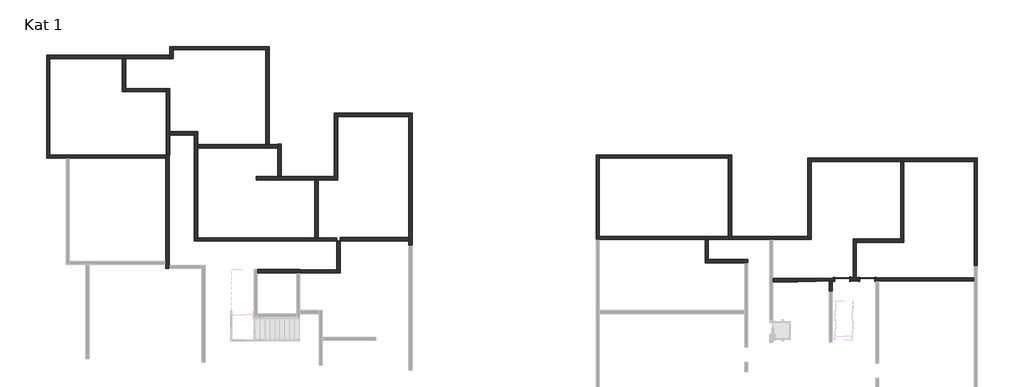
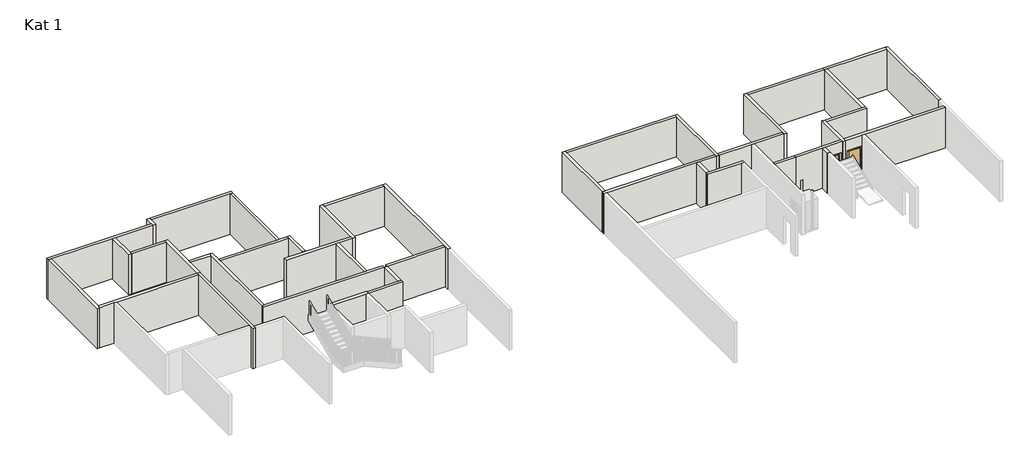
# One storey, part 2 of 3: 43 walls, 2 doors.
"""IFC4 building model written with IfcOpenShell, lengths in millimetres."""

import ifcopenshell
import ifcopenshell.guid

model = None  # the IFC model being written
_history = None  # IfcOwnerHistory: only IFC2X3 demands one
_inside = {}  # id of a spatial element -> (the spatial element, [elements in it])
_under = {}  # id of a project, library or spatial element -> (it, [spatial elements below it])
_declared = {}  # id of a project -> (the project, [libraries it declares])
_typed = {}  # id of a type object -> (the type object, [elements of that type])
_made_of = {}  # id of a material, layer set ... -> (it, [elements and type objects made of it])


def new_model(schema):
    """Start an empty IFC model of exactly this schema.

    Asked for "IFC4X3", IfcOpenShell would pick the latest addendum, in which some entities
    have other attributes; the version numbers below select the first issue.
    IFC2X3 requires an IfcOwnerHistory on every rooted entity: one is made here for all.
    """
    global model, _history
    if schema == "IFC4X3":
        model = ifcopenshell.file(schema_version=(4, 3, 0, 0))
    else:
        model = ifcopenshell.file(schema=schema)
    _inside.clear()
    _under.clear()
    _declared.clear()
    _typed.clear()
    _made_of.clear()
    _history = None
    if model.schema == "IFC2X3":
        org = make("IfcOrganization", Name="unknown")
        user = make(
            "IfcPersonAndOrganization",
            ThePerson=make("IfcPerson", FamilyName="unknown"),
            TheOrganization=org,
        )
        app = make(
            "IfcApplication",
            ApplicationDeveloper=org,
            Version="unknown",
            ApplicationFullName="unknown",
            ApplicationIdentifier="unknown",
        )
        _history = make(
            "IfcOwnerHistory",
            OwningUser=user,
            OwningApplication=app,
            ChangeAction="ADDED",
            CreationDate=0,
        )
    return model


def make(cls, **values):
    """One entity of the class cls with the attributes given. An attribute that is None is left unset."""
    return model.create_entity(
        cls, **{name: value for name, value in values.items() if value is not None}
    )


def rooted(cls, **values):
    """An entity with a GlobalId (a new one), such as an element, a storey or a relation."""
    return make(cls, GlobalId=ifcopenshell.guid.new(), OwnerHistory=_history, **values)


def si_unit(unit_type, name, prefix=None):
    """IfcSIUnit, for example si_unit("LENGTHUNIT", "METRE", prefix="MILLI")."""
    return make("IfcSIUnit", UnitType=unit_type, Prefix=prefix, Name=name)


def assignment(units):
    """IfcUnitAssignment: the units of a project."""
    return None if units is None else make("IfcUnitAssignment", Units=units)


def point(xyz):
    """IfcCartesianPoint."""
    return None if xyz is None else make("IfcCartesianPoint", Coordinates=xyz)


def direction(xyz):
    """IfcDirection."""
    return None if xyz is None else make("IfcDirection", DirectionRatios=xyz)


def frame(location, z_axis=None, x_axis=None):
    """IfcAxis2Placement3D, a coordinate frame: its origin and axes. An axis left out is left unset."""
    return make(
        "IfcAxis2Placement3D",
        Location=point(location),
        Axis=direction(z_axis),
        RefDirection=direction(x_axis),
    )


def origin():
    """The frame at (0, 0, 0) with its axes left unset."""
    return frame((0.0, 0.0, 0.0))


def origin_with_axes():
    """The frame at (0, 0, 0) with the z axis (0, 0, 1) and the x axis (1, 0, 0) written out."""
    return frame((0.0, 0.0, 0.0), z_axis=(0.0, 0.0, 1.0), x_axis=(1.0, 0.0, 0.0))


def place(relative_to, where):
    """IfcLocalPlacement: puts the frame where relative to a parent placement (None: the world)."""
    return make(
        "IfcLocalPlacement", PlacementRelTo=relative_to, RelativePlacement=where
    )


def context(
    kind, dimensions, precision=None, world=None, true_north=None, identifier=None
):
    """IfcGeometricRepresentationContext, for example the 3D "Model" context."""
    return make(
        "IfcGeometricRepresentationContext",
        ContextIdentifier=identifier,
        ContextType=kind,
        CoordinateSpaceDimension=dimensions,
        Precision=precision,
        WorldCoordinateSystem=world,
        TrueNorth=true_north,
    )


def project(units=None, contexts=None):
    """IfcProject with its units and contexts."""
    return rooted(
        "IfcProject",
        Name="project",
        RepresentationContexts=contexts,
        UnitsInContext=assignment(units),
    )


def spatial(cls, under=None, at=None, **own):
    """A site, building, storey or space (cls), placed at a placement, below another one or the project."""
    s = rooted(cls, ObjectPlacement=at, **own)
    if under is not None:
        _under.setdefault(under.id(), (under, []))[1].append(s)
    return s


def polyline(points):
    """IfcPolyline through the points."""
    return make("IfcPolyline", Points=[point(p) for p in points])


def outline(outer, holes=None, kind="AREA"):
    """IfcArbitraryClosedProfileDef: a profile drawn as a closed curve; with holes, ...WithVoids."""
    if holes is None:
        return make("IfcArbitraryClosedProfileDef", ProfileType=kind, OuterCurve=outer)
    return make(
        "IfcArbitraryProfileDefWithVoids",
        ProfileType=kind,
        OuterCurve=outer,
        InnerCurves=holes,
    )


def extrude(swept, where, along, depth):
    """IfcExtrudedAreaSolid: the profile swept, set in the frame where, extruded along a direction by depth."""
    return make(
        "IfcExtrudedAreaSolid",
        SweptArea=swept,
        Position=where,
        ExtrudedDirection=direction(along),
        Depth=depth,
    )


def faces_of(points, faces, orient=None, outer=None):
    """IfcFace entities. A face is a list of loops; a loop is a list of indices into points, from 0.

    orient and outer hold one flag for each loop. By default every Orientation is true, the
    first loop of a face is its IfcFaceOuterBound and the others are IfcFaceBound.
    """
    made = []
    for i, loops in enumerate(faces):
        bounds = []
        for j, loop in enumerate(loops):
            is_outer = j == 0 if outer is None else outer[i][j]
            bounds.append(
                make(
                    "IfcFaceOuterBound" if is_outer else "IfcFaceBound",
                    Bound=make("IfcPolyLoop", Polygon=[points[k] for k in loop]),
                    Orientation=True if orient is None else orient[i][j],
                )
            )
        made.append(make("IfcFace", Bounds=bounds))
    return made


def faceted_brep(points, faces, orient=None, outer=None, voids=None):
    """IfcFacetedBrep: a solid bounded by flat faces; with voids (closed shells), ...WithVoids."""
    shared = [point(p) for p in points]
    hull = make("IfcClosedShell", CfsFaces=faces_of(shared, faces, orient, outer))
    if voids is None:
        return make("IfcFacetedBrep", Outer=hull)
    return make(
        "IfcFacetedBrepWithVoids",
        Outer=hull,
        Voids=[
            make(cls, CfsFaces=faces_of(shared, fs, o, b)) for cls, fs, o, b in voids
        ],
    )


def shape(context_of_items, identifier, shape_type, items):
    """IfcShapeRepresentation: the items that make up one representation, for example the "Body"."""
    return make(
        "IfcShapeRepresentation",
        ContextOfItems=context_of_items,
        RepresentationIdentifier=identifier,
        RepresentationType=shape_type,
        Items=items,
    )


def source(mapping_origin, context_of_items, identifier, shape_type, items):
    """IfcRepresentationMap: a shape defined once, which mapped items show again and again."""
    return make(
        "IfcRepresentationMap",
        MappingOrigin=mapping_origin,
        MappedRepresentation=shape(context_of_items, identifier, shape_type, items),
    )


def transform(
    local_origin,
    x_axis=None,
    y_axis=None,
    z_axis=None,
    scale=None,
    scale2=None,
    scale3=None,
    uniform=True,
):
    """IfcCartesianTransformationOperator3D, or its non-uniform kind. x_axis, y_axis, z_axis: its Axis1, 2, 3."""
    if uniform:
        return make(
            "IfcCartesianTransformationOperator3D",
            Axis1=direction(x_axis),
            Axis2=direction(y_axis),
            LocalOrigin=point(local_origin),
            Scale=scale,
            Axis3=direction(z_axis),
        )
    return make(
        "IfcCartesianTransformationOperator3DnonUniform",
        Axis1=direction(x_axis),
        Axis2=direction(y_axis),
        LocalOrigin=point(local_origin),
        Scale=scale,
        Axis3=direction(z_axis),
        Scale2=scale2,
        Scale3=scale3,
    )


def mapped(mapping_source, mapping_target):
    """IfcMappedItem: shows the shape of a source again, moved by a transform."""
    return make(
        "IfcMappedItem", MappingSource=mapping_source, MappingTarget=mapping_target
    )


def made_of(thing, what):
    """Note that an element or type object is made of a material, layer set ...; save() writes the relation."""
    if what is not None:
        _made_of.setdefault(what.id(), (what, []))[1].append(thing)
    return thing


def element(
    cls,
    number,
    at=None,
    inside=None,
    cuts=None,
    type_object=None,
    material=None,
    context=None,
    identifier="Body",
    shape_type=None,
    held_by="IfcProductDefinitionShape",
    body=None,
    shapes=None,
    **own,
):
    """One element of the class cls, such as IfcWall. Its Tag is "e" and its number.

    at: its placement. inside: the storey or other place that contains it. cuts: it is an
    opening in that element (IfcRelVoidsElement). A single representation is given by context,
    identifier, shape_type and body (its items); several are given by shapes. held_by: the class
    of the entity that holds the representations. save() writes the other relations.
    """
    e = rooted(cls, Tag="e%d" % number, ObjectPlacement=at, **own)
    if body is not None:
        shapes = [shape(context, identifier, shape_type, body)]
    if shapes is not None:
        e.Representation = make(held_by, Representations=shapes)
    if inside is not None:
        _inside.setdefault(inside.id(), (inside, []))[1].append(e)
    if cuts is not None:
        rooted(
            "IfcRelVoidsElement", RelatingBuildingElement=cuts, RelatedOpeningElement=e
        )
    if type_object is not None:
        _typed.setdefault(type_object.id(), (type_object, []))[1].append(e)
    return made_of(e, material)


def aggregate(whole, parts):
    """IfcRelAggregates: a whole, such as a stair, and the parts it consists of."""
    return rooted("IfcRelAggregates", RelatingObject=whole, RelatedObjects=parts)


def save(model, path):
    """Write the relations noted so far, then the file.

    IfcRelAggregates (storeys below a building ...), IfcRelContainedInSpatialStructure (elements
    in a storey), IfcRelDefinesByType, IfcRelAssociatesMaterial and IfcRelDeclares: one each for
    every whole, place, type object, material and project.
    """
    for whole, parts in _under.values():
        aggregate(whole, parts)
    for where, things in _inside.values():
        rooted(
            "IfcRelContainedInSpatialStructure",
            RelatedElements=things,
            RelatingStructure=where,
        )
    for kind, things in _typed.values():
        rooted("IfcRelDefinesByType", RelatedObjects=things, RelatingType=kind)
    for what, things in _made_of.values():
        rooted("IfcRelAssociatesMaterial", RelatedObjects=things, RelatingMaterial=what)
    for by, libraries in _declared.values():
        rooted("IfcRelDeclares", RelatingContext=by, RelatedDefinitions=libraries)
    model.write(path)


def m_single_flush_0915_x_2134mm_727434cd(model_context):
    return source(origin(), model_context, "Body", "SweptSolid", [
        extrude(outline(polyline([(2210.0, -533.5), (0.0, -533.5), (0.0, -457.5), (2134.0, -457.5), (2134.0, 457.5), (0.0, 457.5), (0.0, 533.5), (2210.0, 533.5), (2210.0, -533.5)])), frame((0.0, -125.0, 0.0), z_axis=(0.0, 1.0, 0.0), x_axis=(0.0, 0.0, 1.0)), (0.0, 0.0, 1.0), 25.0),
        extrude(outline(polyline([(2210.0, 533.5), (2210.0, -533.5), (0.0, -533.5), (0.0, -457.5), (2134.0, -457.5), (2134.0, 457.5), (0.0, 457.5), (0.0, 533.5), (2210.0, 533.5)])), frame((0.0, 100.0, 0.0), z_axis=(0.0, 1.0, 0.0), x_axis=(0.0, 0.0, 1.0)), (0.0, 0.0, 1.0), 25.0),
        extrude(outline(polyline([(457.5, -49.0), (457.5, -100.0), (-457.5, -100.0), (-457.5, -49.0), (457.5, -49.0)])), origin_with_axes(), (0.0, 0.0, 1.0), 2134.0),
    ])


def m_single_flush_0915_x_2134mm_6a9e8738(model_context):
    return source(origin(), model_context, "Body", "SweptSolid", [
        extrude(outline(polyline([(2210.0, -533.5), (0.0, -533.5), (0.0, -457.5), (2134.0, -457.5), (2134.0, 457.5), (0.0, 457.5), (0.0, 533.5), (2210.0, 533.5), (2210.0, -533.5)])), frame((0.0, 100.0, 0.0), z_axis=(0.0, 1.0, 0.0), x_axis=(0.0, 0.0, 1.0)), (0.0, 0.0, 1.0), 25.0),
        extrude(outline(polyline([(2210.0, 533.5), (2210.0, -533.5), (0.0, -533.5), (0.0, -457.5), (2134.0, -457.5), (2134.0, 457.5), (0.0, 457.5), (0.0, 533.5), (2210.0, 533.5)])), frame((0.0, -125.0, 0.0), z_axis=(0.0, 1.0, 0.0), x_axis=(0.0, 0.0, 1.0)), (0.0, 0.0, 1.0), 25.0),
        extrude(outline(polyline([(457.5, 49.0), (-457.5, 49.0), (-457.5, 100.0), (457.5, 100.0), (457.5, 49.0)])), origin_with_axes(), (0.0, 0.0, 1.0), 2134.0),
    ])


model = new_model("IFC4")

# Units and contexts
model_context = context("Model", 3, world=origin())
ifc_project = project(units=[si_unit("LENGTHUNIT", "METRE", prefix="MILLI")], contexts=[model_context])

# Site, building, storey
site = spatial("IfcSite", under=ifc_project)
building = spatial("IfcBuilding", under=site)
storey = spatial("IfcBuildingStorey", under=building, Name="Kat 1", Elevation=3000.0)

# Doors
placement = place(None, origin())
m_single_flush_0915_x_2134mm_shape = m_single_flush_0915_x_2134mm_727434cd(model_context)
element("IfcDoor", 1, ObjectType="M_Single-Flush : 0915 x 2134mm", at=placement, inside=storey, context=model_context, shape_type="MappedRepresentation", body=[
    mapped(m_single_flush_0915_x_2134mm_shape, transform((23647.336337, 521.2707349, 3000.0), x_axis=(-1.0, 0.0, 0.0), y_axis=(0.0, -1.0, 0.0), z_axis=(0.0, 0.0, 1.0))),
])
m_single_flush_0915_x_2134mm_2_shape = m_single_flush_0915_x_2134mm_6a9e8738(model_context)
element("IfcDoor", 2, ObjectType="M_Single-Flush : 0915 x 2134mm", at=placement, inside=storey, context=model_context, shape_type="MappedRepresentation", body=[
    mapped(m_single_flush_0915_x_2134mm_2_shape, transform((22134.1969486, 528.0657675, 3000.0), x_axis=(0.9998476951563913, 0.01745240643728349, 0.0), y_axis=(-0.01745240643728349, 0.9998476951563913, 0.0), z_axis=(0.0, 0.0, 1.0))),
])

# Walls
element("IfcWall", 3, ObjectType="Generic - 200mm", at=placement, inside=storey, context=model_context, shape_type="Brep", body=[
    faceted_brep([(25649.836337, 7621.2707349, 3000.0), (25849.836337, 7621.2707349, 3000.0), (30068.3425199, 7621.2707349, 3000.0), (30068.3425199, 7621.2707349, 6000.0), (25849.836337, 7621.2707349, 6000.0), (25649.836337, 7621.2707349, 6000.0), (25649.836337, 7821.2707349, 3000.0), (25649.836337, 7821.2707349, 6000.0), (30068.3425199, 7821.2707349, 6000.0), (30068.3425199, 7821.2707349, 3000.0), (30068.3425199, 7819.475628, 3000.0)], [[[0, 1, 2, 3, 4, 5]], [[6, 7, 8, 9]], [[2, 1, 0, 6, 9, 10]], [[5, 4, 3, 8, 7]], [[0, 5, 7, 6]], [[3, 2, 10, 9, 8]]]),
])
element("IfcWall", 4, ObjectType="Generic - 200mm", at=placement, inside=storey, context=model_context, shape_type="Brep", body=[
    faceted_brep([(30068.3425199, 7821.2707349, 3000.0), (30068.3425199, 7819.475628, 3000.0), (30068.3425199, 7621.2707349, 3000.0), (30068.3425199, 1319.475628, 3000.0), (30068.3425199, 1319.475628, 6000.0), (30068.3425199, 7621.2707349, 6000.0), (30068.3425199, 7821.2707349, 6000.0), (30268.3425199, 7821.2707349, 3000.0), (30268.3425199, 7821.2707349, 6000.0), (30268.3425199, 1319.475628, 6000.0), (30268.3425199, 1319.475628, 3000.0), (30268.3425199, 7819.475628, 3000.0), (30068.8612349, 1319.475628, 3000.0), (30068.8612349, 1319.475628, 6000.0)], [[[0, 1, 2, 3, 4, 5, 6]], [[7, 8, 9, 10, 11]], [[3, 2, 1, 0, 7, 11, 10, 12]], [[4, 3, 12, 10, 9, 13]], [[6, 5, 4, 13, 9, 8]], [[0, 6, 8, 7]]]),
])
element("IfcWall", 5, ObjectType="Generic - 200mm", at=placement, inside=storey, context=model_context, shape_type="Brep", body=[
    faceted_brep([(21549.836337, -200.524372, 3000.0), (21549.836337, 379.475628, 3000.0), (21549.836337, 417.8504823, 3000.0), (21549.836337, 417.8504823, 6000.0), (21549.836337, -200.524372, 6000.0), (21349.836337, -200.524372, 3000.0), (21349.836337, -200.524372, 6000.0), (21349.836337, 414.3594693, 6000.0), (21349.836337, 414.3594693, 3000.0), (21349.836337, 379.475628, 3000.0)], [[[0, 1, 2, 3, 4]], [[5, 6, 7, 8, 9]], [[2, 1, 0, 5, 9, 8]], [[4, 3, 7, 6]], [[0, 4, 6, 5]], [[3, 2, 8, 7]]]),
])
element("IfcWall", 6, ObjectType="Generic - 200mm", at=placement, inside=storey, context=model_context, shape_type="Brep", body=[
    faceted_brep([(20268.8612349, 7621.2707349, 3000.0), (25649.836337, 7621.2707349, 3000.0), (25649.836337, 7621.2707349, 6000.0), (20268.8612349, 7621.2707349, 6000.0), (20268.8612349, 7821.2707349, 3000.0), (20268.8612349, 7821.2707349, 6000.0), (25649.836337, 7821.2707349, 6000.0), (25649.836337, 7821.2707349, 3000.0), (20268.8612349, 7819.475628, 3000.0)], [[[0, 1, 2, 3]], [[4, 5, 6, 7]], [[1, 0, 8, 4, 7]], [[3, 2, 6, 5]], [[2, 1, 7, 6]], [[0, 3, 5, 4, 8]]]),
])
element("IfcWall", 7, ObjectType="Generic - 200mm", at=placement, inside=storey, context=model_context, shape_type="Brep", body=[
    faceted_brep([(22989.836337, 421.2707349, 3000.0), (22989.836337, 621.2707349, 3000.0), (22989.836337, 2756.2707349, 3000.0), (22989.836337, 2956.2707349, 3000.0), (22989.836337, 2956.2707349, 6000.0), (22989.836337, 2756.2707349, 6000.0), (22989.836337, 621.2707349, 6000.0), (22989.836337, 421.2707349, 6000.0), (22789.836337, 421.2707349, 3000.0), (22789.836337, 421.2707349, 6000.0), (22789.836337, 439.4947628, 6000.0), (22789.836337, 639.5252284, 6000.0), (22789.836337, 2956.2707349, 6000.0), (22789.836337, 2956.2707349, 3000.0), (22789.836337, 639.5252284, 3000.0), (22789.836337, 439.4947628, 3000.0)], [[[0, 1, 2, 3, 4, 5, 6, 7]], [[8, 9, 10, 11, 12, 13, 14, 15]], [[3, 2, 1, 0, 8, 15, 14, 13]], [[7, 6, 5, 4, 12, 11, 10, 9]], [[4, 3, 13, 12]], [[0, 7, 9, 8]]]),
])
element("IfcWall", 8, ObjectType="Generic - 200mm", at=placement, inside=storey, context=model_context, shape_type="Brep", body=[
    faceted_brep([(13888.8612349, 1521.4230978, 3000.0), (16270.6041014, 1521.4230978, 3000.0), (16470.6041014, 1521.4230978, 3000.0), (16470.6041014, 1521.4230978, 6000.0), (16270.6041014, 1521.4230978, 6000.0), (13888.8612349, 1521.4230978, 6000.0), (13888.8612349, 1721.4230978, 3000.0), (13888.8612349, 1721.4230978, 6000.0), (14088.8612349, 1721.4230978, 6000.0), (16470.6041014, 1721.4230978, 6000.0), (16470.6041014, 1721.4230978, 3000.0), (14088.8612349, 1721.4230978, 3000.0)], [[[0, 1, 2, 3, 4, 5]], [[6, 7, 8, 9, 10, 11]], [[2, 1, 0, 6, 11, 10]], [[5, 4, 3, 9, 8, 7]], [[0, 5, 7, 6]], [[3, 2, 10, 9]]]),
])
element("IfcWall", 9, ObjectType="Generic - 200mm", at=placement, inside=storey, context=model_context, shape_type="Brep", body=[
    faceted_brep([(20068.8612349, 7821.2707349, 3000.0), (20068.8612349, 7819.475628, 3000.0), (20068.8612349, 3121.2707349, 3000.0), (20068.8612349, 2921.2707349, 3000.0), (20068.8612349, 2921.2707349, 6000.0), (20068.8612349, 3121.2707349, 6000.0), (20068.8612349, 7821.2707349, 6000.0), (20268.8612349, 7821.2707349, 3000.0), (20268.8612349, 7821.2707349, 6000.0), (20268.8612349, 7621.2707349, 6000.0), (20268.8612349, 2921.2707349, 6000.0), (20268.8612349, 2921.2707349, 3000.0), (20268.8612349, 7621.2707349, 3000.0), (20268.8612349, 7819.475628, 3000.0)], [[[0, 1, 2, 3, 4, 5, 6]], [[7, 8, 9, 10, 11, 12, 13]], [[3, 2, 1, 0, 7, 13, 12, 11]], [[6, 5, 4, 10, 9, 8]], [[0, 6, 8, 7]], [[4, 3, 11, 10]]]),
])
element("IfcWall", 10, ObjectType="Generic - 200mm", at=placement, inside=storey, context=model_context, shape_type="Brep", body=[
    faceted_brep([(30068.8612349, 421.2707349, 6000.0), (24348.8612349, 421.2707349, 6000.0), (24148.8612349, 421.2707349, 6000.0), (22989.836337, 421.2707349, 6000.0), (22989.836337, 421.2707349, 3000.0), (23189.836337, 421.2707349, 3000.0), (23189.836337, 421.2707349, 5134.0), (24104.836337, 421.2707349, 5134.0), (24104.836337, 421.2707349, 3000.0), (24148.8612349, 421.2707349, 3000.0), (24348.8612349, 421.2707349, 3000.0), (30068.8612349, 421.2707349, 3000.0), (22989.836337, 621.2707349, 6000.0), (30068.8612349, 621.2707349, 6000.0), (30068.8612349, 621.2707349, 3000.0), (24104.836337, 621.2707349, 3000.0), (24104.836337, 621.2707349, 5134.0), (23189.836337, 621.2707349, 5134.0), (23189.836337, 621.2707349, 3000.0), (22989.836337, 621.2707349, 3000.0)], [[[0, 1, 2, 3, 4, 5, 6, 7, 8, 9, 10, 11]], [[12, 13, 14, 15, 16, 17, 18, 19]], [[14, 11, 10, 9, 8, 15]], [[4, 19, 18, 5]], [[3, 2, 1, 0, 13, 12]], [[0, 11, 14, 13]], [[17, 6, 5, 18]], [[7, 16, 15, 8]], [[16, 7, 6, 17]], [[19, 4, 3, 12]]]),
])
element("IfcWall", 11, ObjectType="Generic - 200mm", at=placement, inside=storey, context=model_context, shape_type="SweptSolid", body=[
    extrude(outline(polyline([(17970.6041014, 581.2707349), (19452.4386392, 581.2707349), (19454.1840127, 381.2707349), (17970.6041014, 381.2707349), (17970.6041014, 581.2707349)])), frame((0.0, 0.0, 3000.0), z_axis=(0.0, 0.0, 1.0), x_axis=(1.0, 0.0, 0.0)), (0.0, 0.0, 1.0), 3000.0),
])
element("IfcWall", 12, ObjectType="Generic - 200mm", at=placement, inside=storey, context=model_context, shape_type="Brep", body=[
    faceted_brep([(19452.4386392, 581.2707349, 6000.0), (22789.836337, 639.5252284, 6000.0), (22789.836337, 639.5252284, 3000.0), (22589.8820285, 636.035013, 3000.0), (22589.8820285, 636.035013, 5134.0), (21675.0213874, 620.0660611, 5134.0), (21675.0213874, 620.0660611, 3000.0), (19452.4386392, 581.2707349, 3000.0), (22789.836337, 439.4947628, 6000.0), (21549.836337, 417.8504823, 6000.0), (21349.836337, 414.3594693, 6000.0), (19454.1840127, 381.2707349, 6000.0), (19454.1840127, 381.2707349, 3000.0), (21349.836337, 414.3594693, 3000.0), (21549.836337, 417.8504823, 3000.0), (21678.5118687, 420.0965221, 3000.0), (21678.5118687, 420.0965221, 5134.0), (22593.3725098, 436.0654739, 5134.0), (22593.3725098, 436.0654739, 3000.0), (22789.836337, 439.4947628, 3000.0)], [[[0, 1, 2, 3, 4, 5, 6, 7]], [[8, 9, 10, 11, 12, 13, 14, 15, 16, 17, 18, 19]], [[2, 19, 18, 3]], [[12, 7, 6, 15, 14, 13]], [[1, 0, 11, 10, 9, 8]], [[17, 4, 3, 18]], [[5, 16, 15, 6]], [[16, 5, 4, 17]], [[2, 1, 8, 19]], [[11, 0, 7, 12]]]),
])
element("IfcWall", 13, ObjectType="Generic - 200mm", at=placement, inside=storey, context=model_context, shape_type="Brep", body=[
    faceted_brep([(22989.836337, 2756.2707349, 3000.0), (25849.836337, 2756.2707349, 3000.0), (25849.836337, 2756.2707349, 6000.0), (22989.836337, 2756.2707349, 6000.0), (22989.836337, 2956.2707349, 3000.0), (22989.836337, 2956.2707349, 6000.0), (25649.836337, 2956.2707349, 6000.0), (25849.836337, 2956.2707349, 6000.0), (25849.836337, 2956.2707349, 3000.0), (25649.836337, 2956.2707349, 3000.0)], [[[0, 1, 2, 3]], [[4, 5, 6, 7, 8, 9]], [[1, 0, 4, 9, 8]], [[3, 2, 7, 6, 5]], [[2, 1, 8, 7]], [[0, 3, 5, 4]]]),
])
element("IfcWall", 14, ObjectType="Generic - 200mm", at=placement, inside=storey, context=model_context, shape_type="SweptSolid", body=[
    extrude(outline(polyline([(25849.836337, 7621.2707349), (25849.836337, 2956.2707349), (25649.836337, 2956.2707349), (25649.836337, 7621.2707349), (25849.836337, 7621.2707349)])), frame((0.0, 0.0, 3000.0), z_axis=(0.0, 0.0, 1.0), x_axis=(1.0, 0.0, 0.0)), (0.0, 0.0, 1.0), 3000.0),
])
element("IfcWall", 15, ObjectType="Generic - 200mm", at=placement, inside=storey, context=model_context, shape_type="Brep", body=[
    faceted_brep([(-10469.8304233, 1122.632394, 3000.0), (-13026.101437, 1122.632394, 3000.0), (-13026.101437, 1122.632394, 6000.0), (-10469.8304233, 1122.632394, 6000.0), (-10469.8304233, 922.632394, 3000.0), (-10469.8304233, 922.632394, 6000.0), (-10669.8304233, 922.632394, 6000.0), (-13026.101437, 922.632394, 6000.0), (-13026.101437, 922.632394, 3000.0), (-10669.8304233, 922.632394, 3000.0), (-10469.8304233, 1102.632394, 3000.0), (-13026.101437, 1120.8372871, 3000.0), (-10469.8304233, 1102.632394, 6000.0)], [[[0, 1, 2, 3]], [[4, 5, 6, 7, 8, 9]], [[1, 0, 10, 4, 9, 8, 11]], [[3, 2, 7, 6, 5, 12]], [[0, 3, 12, 5, 4, 10]], [[2, 1, 11, 8, 7]]]),
])
element("IfcWall", 16, ObjectType="Generic - 200mm", at=placement, inside=storey, context=model_context, shape_type="Brep", body=[
    faceted_brep([(-18289.8304233, 8014.6351355, 3000.0), (-18289.8304233, 9214.6351355, 3000.0), (-18289.8304233, 9414.6351355, 3000.0), (-18289.8304233, 12014.6351355, 3000.0), (-18289.8304233, 12014.6351355, 6000.0), (-18289.8304233, 9414.6351355, 6000.0), (-18289.8304233, 9214.6351355, 6000.0), (-18289.8304233, 8014.6351355, 6000.0), (-18489.8304233, 8014.6351355, 3000.0), (-18489.8304233, 8014.6351355, 6000.0), (-18489.8304233, 11814.6351355, 6000.0), (-18489.8304233, 12014.6351355, 6000.0), (-18489.8304233, 12014.6351355, 3000.0), (-18489.8304233, 11814.6351355, 3000.0), (-18323.9741722, 8014.6351355, 3000.0), (-18323.9741722, 8014.6351355, 6000.0)], [[[0, 1, 2, 3, 4, 5, 6, 7]], [[8, 9, 10, 11, 12, 13]], [[3, 2, 1, 0, 14, 8, 13, 12]], [[7, 6, 5, 4, 11, 10, 9, 15]], [[0, 7, 15, 9, 8, 14]], [[4, 3, 12, 11]]]),
])
element("IfcWall", 17, ObjectType="Generic - 200mm", at=placement, inside=storey, context=model_context, shape_type="Brep", body=[
    faceted_brep([(15288.8612349, 3120.535295, 3000.0), (7543.716007, 3120.535295, 3000.0), (7343.716007, 3120.535295, 3000.0), (7343.716007, 3120.535295, 6000.0), (7543.716007, 3120.535295, 6000.0), (15288.8612349, 3120.535295, 6000.0), (15288.8612349, 2920.535295, 3000.0), (15288.8612349, 2920.535295, 6000.0), (14088.8612349, 2920.535295, 6000.0), (13888.8612349, 2920.535295, 6000.0), (7543.716007, 2920.535295, 6000.0), (7343.716007, 2920.535295, 6000.0), (7343.716007, 2920.535295, 3000.0), (7543.716007, 2920.535295, 3000.0), (13888.8612349, 2920.535295, 3000.0), (14088.8612349, 2920.535295, 3000.0), (7343.716007, 3020.535295, 3000.0)], [[[0, 1, 2, 3, 4, 5]], [[6, 7, 8, 9, 10, 11, 12, 13, 14, 15]], [[2, 1, 0, 6, 15, 14, 13, 12, 16]], [[5, 4, 3, 11, 10, 9, 8, 7]], [[3, 2, 16, 12, 11]], [[0, 5, 7, 6]]]),
])
element("IfcWall", 18, ObjectType="Generic - 200mm", at=placement, inside=storey, context=model_context, shape_type="Brep", body=[
    faceted_brep([(-12326.101437, 14542.632394, 3000.0), (-18089.8304233, 14542.632394, 3000.0), (-18089.8304233, 14542.632394, 6000.0), (-12326.101437, 14542.632394, 6000.0), (-12326.101437, 14342.632394, 3000.0), (-12326.101437, 14342.632394, 6000.0), (-12526.101437, 14342.632394, 6000.0), (-18089.8304233, 14342.632394, 6000.0), (-18089.8304233, 14342.632394, 3000.0), (-12526.101437, 14342.632394, 3000.0), (-12326.101437, 14540.8372871, 3000.0), (-18089.8304233, 14540.8372871, 3000.0)], [[[0, 1, 2, 3]], [[4, 5, 6, 7, 8, 9]], [[1, 0, 10, 4, 9, 8, 11]], [[3, 2, 7, 6, 5]], [[2, 1, 11, 8, 7]], [[0, 3, 5, 4, 10]]]),
])
element("IfcWall", 19, ObjectType="Generic - 200mm", at=placement, inside=storey, context=model_context, shape_type="Brep", body=[
    faceted_brep([(-25701.4369496, 13814.6351355, 3000.0), (-25701.4369496, 13812.8400285, 3000.0), (-25701.4369496, 7814.6351355, 3000.0), (-25701.4369496, 7814.6351355, 6000.0), (-25701.4369496, 13814.6351355, 6000.0), (-25501.4369496, 13814.6351355, 3000.0), (-25501.4369496, 13814.6351355, 6000.0), (-25501.4369496, 8014.6351355, 6000.0), (-25501.4369496, 7814.6351355, 6000.0), (-25501.4369496, 7814.6351355, 3000.0), (-25501.4369496, 8014.6351355, 3000.0), (-25501.4369496, 13812.8400285, 3000.0)], [[[0, 1, 2, 3, 4]], [[5, 6, 7, 8, 9, 10, 11]], [[2, 1, 0, 5, 11, 10, 9]], [[4, 3, 8, 7, 6]], [[3, 2, 9, 8]], [[0, 4, 6, 5]]]),
])
element("IfcWall", 20, ObjectType="Generic - 200mm", at=placement, inside=storey, context=model_context, shape_type="Brep", body=[
    faceted_brep([(-25501.4369496, 7814.6351355, 3000.0), (-24523.9741722, 7814.6351355, 3000.0), (-24323.9741722, 7814.6351355, 3000.0), (-18523.9741722, 7814.6351355, 3000.0), (-18523.9741722, 7814.6351355, 6000.0), (-24323.9741722, 7814.6351355, 6000.0), (-24523.9741722, 7814.6351355, 6000.0), (-25501.4369496, 7814.6351355, 6000.0), (-25501.4369496, 8014.6351355, 3000.0), (-25501.4369496, 8014.6351355, 6000.0), (-18523.9741722, 8014.6351355, 6000.0), (-18523.9741722, 8014.6351355, 3000.0), (-25501.4369496, 8012.8400285, 3000.0)], [[[0, 1, 2, 3, 4, 5, 6, 7]], [[8, 9, 10, 11]], [[3, 2, 1, 0, 12, 8, 11]], [[7, 6, 5, 4, 10, 9]], [[4, 3, 11, 10]], [[0, 7, 9, 8, 12]]]),
])
element("IfcWall", 21, ObjectType="Generic - 200mm", at=placement, inside=storey, context=model_context, shape_type="Brep", body=[
    faceted_brep([(-18289.8304233, 14014.6351355, 3000.0), (-25701.4369496, 14014.6351355, 3000.0), (-25701.4369496, 14014.6351355, 6000.0), (-18289.8304233, 14014.6351355, 6000.0), (-18289.8304233, 13814.6351355, 3000.0), (-18289.8304233, 13814.6351355, 6000.0), (-20949.8304233, 13814.6351355, 6000.0), (-21149.8304233, 13814.6351355, 6000.0), (-25501.4369496, 13814.6351355, 6000.0), (-25701.4369496, 13814.6351355, 6000.0), (-25701.4369496, 13814.6351355, 3000.0), (-25501.4369496, 13814.6351355, 3000.0), (-21149.8304233, 13814.6351355, 3000.0), (-20949.8304233, 13814.6351355, 3000.0), (-18289.8304233, 14012.8400285, 3000.0), (-25701.4369496, 14012.8400285, 3000.0)], [[[0, 1, 2, 3]], [[4, 5, 6, 7, 8, 9, 10, 11, 12, 13]], [[1, 0, 14, 4, 13, 12, 11, 10, 15]], [[3, 2, 9, 8, 7, 6, 5]], [[2, 1, 15, 10, 9]], [[0, 3, 5, 4, 14]]]),
])
element("IfcWall", 22, ObjectType="Generic - 200mm", at=placement, inside=storey, context=model_context, shape_type="SweptSolid", body=[
    extrude(outline(polyline([(-16823.9741722, 9214.6351355), (-18289.8304233, 9214.6351355), (-18289.8304233, 9414.6351355), (-16823.9741722, 9414.6351355), (-16823.9741722, 9214.6351355)])), frame((0.0, 0.0, 3000.0), z_axis=(0.0, 0.0, 1.0), x_axis=(1.0, 0.0, 0.0)), (0.0, 0.0, 1.0), 3000.0),
])
element("IfcWall", 23, ObjectType="Generic - 200mm", at=placement, inside=storey, context=model_context, shape_type="Brep", body=[
    faceted_brep([(-18523.9741722, 8014.6351355, 3000.0), (-18523.9741722, 7814.6351355, 3000.0), (-18523.9741722, 1614.6351355, 3000.0), (-18523.9741722, 1414.6351355, 3000.0), (-18523.9741722, 1174.6351355, 3000.0), (-18523.9741722, 1174.6351355, 6000.0), (-18523.9741722, 1414.6351355, 6000.0), (-18523.9741722, 1614.6351355, 6000.0), (-18523.9741722, 7814.6351355, 6000.0), (-18523.9741722, 8014.6351355, 6000.0), (-18323.9741722, 8014.6351355, 3000.0), (-18323.9741722, 8014.6351355, 6000.0), (-18323.9741722, 1374.6351355, 6000.0), (-18323.9741722, 1174.6351355, 6000.0), (-18323.9741722, 1174.6351355, 3000.0), (-18323.9741722, 1374.6351355, 3000.0), (-18489.8304233, 8014.6351355, 3000.0), (-18489.8304233, 8014.6351355, 6000.0)], [[[0, 1, 2, 3, 4, 5, 6, 7, 8, 9]], [[10, 11, 12, 13, 14, 15]], [[4, 3, 2, 1, 0, 16, 10, 15, 14]], [[9, 8, 7, 6, 5, 13, 12, 11, 17]], [[0, 9, 17, 11, 10, 16]], [[5, 4, 14, 13]]]),
])
element("IfcWall", 24, ObjectType="Generic - 200mm", at=placement, inside=storey, context=model_context, shape_type="SweptSolid", body=[
    extrude(outline(polyline([(-9570.3449834, 3022.632394), (-9570.3449834, 6502.632394), (-9370.3449834, 6502.632394), (-9370.3449834, 3022.632394), (-9570.3449834, 3022.632394)])), frame((0.0, 0.0, 3000.0), z_axis=(0.0, 0.0, 1.0), x_axis=(1.0, 0.0, 0.0)), (0.0, 0.0, 1.0), 3000.0),
])
element("IfcWall", 25, ObjectType="Generic - 200mm", at=placement, inside=storey, context=model_context, shape_type="Brep", body=[
    faceted_brep([(-16623.9741722, 3022.632394, 3000.0), (-16623.9741722, 8442.632394, 3000.0), (-16623.9741722, 8642.632394, 3000.0), (-16623.9741722, 9414.6351355, 3000.0), (-16623.9741722, 9414.6351355, 6000.0), (-16623.9741722, 8642.632394, 6000.0), (-16623.9741722, 8442.632394, 6000.0), (-16623.9741722, 3022.632394, 6000.0), (-16823.9741722, 3022.632394, 3000.0), (-16823.9741722, 3022.632394, 6000.0), (-16823.9741722, 9214.6351355, 6000.0), (-16823.9741722, 9414.6351355, 6000.0), (-16823.9741722, 9414.6351355, 3000.0), (-16823.9741722, 9214.6351355, 3000.0)], [[[0, 1, 2, 3, 4, 5, 6, 7]], [[8, 9, 10, 11, 12, 13]], [[3, 2, 1, 0, 8, 13, 12]], [[7, 6, 5, 4, 11, 10, 9]], [[4, 3, 12, 11]], [[0, 7, 9, 8]]]),
])
element("IfcWall", 26, ObjectType="Generic - 200mm", at=placement, inside=storey, context=model_context, shape_type="Brep", body=[
    faceted_brep([(-8390.3449834, 6702.632394, 3000.0), (-13086.101437, 6702.632394, 3000.0), (-13086.101437, 6702.632394, 6000.0), (-8390.3449834, 6702.632394, 6000.0), (-8390.3449834, 6502.632394, 3000.0), (-8390.3449834, 6502.632394, 6000.0), (-9370.3449834, 6502.632394, 6000.0), (-9570.3449834, 6502.632394, 6000.0), (-13086.101437, 6502.632394, 6000.0), (-13086.101437, 6502.632394, 3000.0), (-9570.3449834, 6502.632394, 3000.0), (-9370.3449834, 6502.632394, 3000.0), (-8390.3449834, 6700.8372871, 3000.0)], [[[0, 1, 2, 3]], [[4, 5, 6, 7, 8, 9, 10, 11]], [[1, 0, 12, 4, 11, 10, 9]], [[2, 1, 9, 8]], [[3, 2, 8, 7, 6, 5]], [[0, 3, 5, 4, 12]]]),
])
element("IfcWall", 27, ObjectType="Generic - 200mm", at=placement, inside=storey, context=model_context, shape_type="Brep", body=[
    faceted_brep([(-16823.9741722, 2822.632394, 3000.0), (-8250.3449834, 2822.632394, 3000.0), (-8240.3449834, 2822.632394, 3000.0), (-8240.3449834, 2822.632394, 6000.0), (-8250.3449834, 2822.632394, 6000.0), (-16823.9741722, 2822.632394, 6000.0), (-16823.9741722, 3022.632394, 3000.0), (-16823.9741722, 3022.632394, 6000.0), (-16623.9741722, 3022.632394, 6000.0), (-9570.3449834, 3022.632394, 6000.0), (-9370.3449834, 3022.632394, 6000.0), (-8240.3449834, 3022.632394, 6000.0), (-8240.3449834, 3022.632394, 3000.0), (-9370.3449834, 3022.632394, 3000.0), (-9570.3449834, 3022.632394, 3000.0), (-16623.9741722, 3022.632394, 3000.0), (-8240.3449834, 2842.632394, 3000.0), (-8240.3449834, 2842.632394, 6000.0)], [[[0, 1, 2, 3, 4, 5]], [[6, 7, 8, 9, 10, 11, 12, 13, 14, 15]], [[2, 1, 0, 6, 15, 14, 13, 12, 16]], [[5, 4, 3, 17, 11, 10, 9, 8, 7]], [[0, 5, 7, 6]], [[3, 2, 16, 12, 11, 17]]]),
])
element("IfcWall", 28, ObjectType="Generic - 200mm", at=placement, inside=storey, context=model_context, shape_type="Brep", body=[
    faceted_brep([(-8050.3449834, 1102.632394, 3000.0), (-8250.3449834, 1102.632394, 3000.0), (-10469.8304233, 1102.632394, 3000.0), (-10469.8304233, 1102.632394, 6000.0), (-8250.3449834, 1102.632394, 6000.0), (-8050.3449834, 1102.632394, 6000.0), (-8050.3449834, 902.632394, 3000.0), (-8050.3449834, 902.632394, 6000.0), (-10469.8304233, 902.632394, 6000.0), (-10469.8304233, 902.632394, 3000.0), (-10469.8304233, 922.632394, 3000.0), (-10469.8304233, 922.632394, 6000.0)], [[[0, 1, 2, 3, 4, 5]], [[6, 7, 8, 9]], [[2, 1, 0, 6, 9, 10]], [[5, 4, 3, 11, 8, 7]], [[3, 2, 10, 9, 8, 11]], [[0, 5, 7, 6]]]),
])
element("IfcWall", 29, ObjectType="Generic - 200mm", at=placement, inside=storey, context=model_context, shape_type="Brep", body=[
    faceted_brep([(-3925.3449834, 10522.632394, 3000.0), (-3925.3449834, 10520.8372871, 3000.0), (-3925.3449834, 10322.632394, 3000.0), (-3925.3449834, 3042.632394, 3000.0), (-3925.3449834, 2842.632394, 3000.0), (-3925.3449834, 2560.8372871, 3000.0), (-3925.3449834, 2560.8372871, 6000.0), (-3925.3449834, 2842.632394, 6000.0), (-3925.3449834, 3042.632394, 6000.0), (-3925.3449834, 10322.632394, 6000.0), (-3925.3449834, 10522.632394, 6000.0), (-3725.3449834, 10522.632394, 3000.0), (-3725.3449834, 10522.632394, 6000.0), (-3725.3449834, 2560.8372871, 6000.0), (-3725.3449834, 2560.8372871, 3000.0), (-3725.3449834, 10520.8372871, 3000.0), (-3920.3449834, 2560.8372871, 3000.0), (-3920.3449834, 2560.8372871, 6000.0)], [[[0, 1, 2, 3, 4, 5, 6, 7, 8, 9, 10]], [[11, 12, 13, 14, 15]], [[5, 4, 3, 2, 1, 0, 11, 15, 14, 16]], [[6, 5, 16, 14, 13, 17]], [[10, 9, 8, 7, 6, 17, 13, 12]], [[0, 10, 12, 11]]]),
])
element("IfcWall", 30, ObjectType="Generic - 200mm", at=placement, inside=storey, context=model_context, shape_type="Brep", body=[
    faceted_brep([(15488.8612349, 2921.2707349, 3000.0), (17770.6041014, 2921.2707349, 3000.0), (17970.6041014, 2921.2707349, 3000.0), (20068.8612349, 2921.2707349, 3000.0), (20068.8612349, 2921.2707349, 6000.0), (17970.6041014, 2921.2707349, 6000.0), (17770.6041014, 2921.2707349, 6000.0), (15488.8612349, 2921.2707349, 6000.0), (15488.8612349, 3121.2707349, 3000.0), (15488.8612349, 3121.2707349, 6000.0), (20068.8612349, 3121.2707349, 6000.0), (20068.8612349, 3121.2707349, 3000.0), (20068.8612349, 3119.475628, 3000.0)], [[[0, 1, 2, 3, 4, 5, 6, 7]], [[8, 9, 10, 11]], [[3, 2, 1, 0, 8, 11, 12]], [[7, 6, 5, 4, 10, 9]], [[0, 7, 9, 8]], [[4, 3, 12, 11, 10]]]),
])
element("IfcWall", 31, ObjectType="Generic - 200mm", at=placement, inside=storey, context=model_context, shape_type="Brep", body=[
    faceted_brep([(7543.716007, 3120.535295, 3000.0), (7543.716007, 7821.2707349, 3000.0), (7543.716007, 8019.475628, 3000.0), (7543.716007, 8021.2707349, 3000.0), (7543.716007, 8021.2707349, 6000.0), (7543.716007, 7821.2707349, 6000.0), (7543.716007, 3120.535295, 6000.0), (7343.716007, 3120.535295, 3000.0), (7343.716007, 3120.535295, 6000.0), (7343.716007, 8021.2707349, 6000.0), (7343.716007, 8021.2707349, 3000.0), (7343.716007, 8019.475628, 3000.0)], [[[0, 1, 2, 3, 4, 5, 6]], [[7, 8, 9, 10, 11]], [[3, 2, 1, 0, 7, 11, 10]], [[6, 5, 4, 9, 8]], [[0, 6, 8, 7]], [[4, 3, 10, 9]]]),
])
element("IfcWall", 32, ObjectType="Generic - 200mm", at=placement, inside=storey, context=model_context, shape_type="Brep", body=[
    faceted_brep([(15488.8612349, 2920.535295, 3000.0), (15488.8612349, 2921.2707349, 3000.0), (15488.8612349, 3121.2707349, 3000.0), (15488.8612349, 8019.475628, 3000.0), (15488.8612349, 8021.2707349, 3000.0), (15488.8612349, 8021.2707349, 6000.0), (15488.8612349, 3121.2707349, 6000.0), (15488.8612349, 2921.2707349, 6000.0), (15488.8612349, 2920.535295, 6000.0), (15288.8612349, 2920.535295, 3000.0), (15288.8612349, 2920.535295, 6000.0), (15288.8612349, 3120.535295, 6000.0), (15288.8612349, 7821.2707349, 6000.0), (15288.8612349, 8021.2707349, 6000.0), (15288.8612349, 8021.2707349, 3000.0), (15288.8612349, 8019.475628, 3000.0), (15288.8612349, 7821.2707349, 3000.0), (15288.8612349, 3120.535295, 3000.0)], [[[0, 1, 2, 3, 4, 5, 6, 7, 8]], [[9, 10, 11, 12, 13, 14, 15, 16, 17]], [[4, 3, 2, 1, 0, 9, 17, 16, 15, 14]], [[8, 7, 6, 5, 13, 12, 11, 10]], [[0, 8, 10, 9]], [[5, 4, 14, 13]]]),
])
element("IfcWall", 33, ObjectType="Generic - 200mm", at=placement, inside=storey, context=model_context, shape_type="Brep", body=[
    faceted_brep([(15288.8612349, 8021.2707349, 3000.0), (7543.716007, 8021.2707349, 3000.0), (7543.716007, 8021.2707349, 6000.0), (15288.8612349, 8021.2707349, 6000.0), (15288.8612349, 7821.2707349, 3000.0), (15288.8612349, 7821.2707349, 6000.0), (7543.716007, 7821.2707349, 6000.0), (7543.716007, 7821.2707349, 3000.0), (15288.8612349, 8019.475628, 3000.0), (7543.716007, 8019.475628, 3000.0)], [[[0, 1, 2, 3]], [[4, 5, 6, 7]], [[1, 0, 8, 4, 7, 9]], [[3, 2, 6, 5]], [[2, 1, 9, 7, 6]], [[0, 3, 5, 4, 8]]]),
])
element("IfcWall", 34, ObjectType="Generic - 200mm", at=placement, inside=storey, context=model_context, shape_type="Brep", body=[
    faceted_brep([(-12526.101437, 14342.632394, 3000.0), (-12526.101437, 14340.8372871, 3000.0), (-12526.101437, 8642.632394, 3000.0), (-12526.101437, 8642.632394, 6000.0), (-12526.101437, 14342.632394, 6000.0), (-12326.101437, 14342.632394, 3000.0), (-12326.101437, 14342.632394, 6000.0), (-12326.101437, 8642.632394, 6000.0), (-12326.101437, 8642.632394, 3000.0), (-12326.101437, 14340.8372871, 3000.0)], [[[0, 1, 2, 3, 4]], [[5, 6, 7, 8, 9]], [[2, 1, 0, 5, 9, 8]], [[4, 3, 7, 6]], [[3, 2, 8, 7]], [[0, 4, 6, 5]]]),
])
element("IfcWall", 35, ObjectType="Generic - 200mm", at=placement, inside=storey, context=model_context, shape_type="Brep", body=[
    faceted_brep([(-11786.101437, 8642.632394, 3000.0), (-12326.101437, 8642.632394, 3000.0), (-12526.101437, 8642.632394, 3000.0), (-16623.9741722, 8642.632394, 3000.0), (-16623.9741722, 8642.632394, 6000.0), (-12526.101437, 8642.632394, 6000.0), (-12326.101437, 8642.632394, 6000.0), (-11786.101437, 8642.632394, 6000.0), (-11786.101437, 8442.632394, 3000.0), (-11786.101437, 8442.632394, 6000.0), (-16623.9741722, 8442.632394, 6000.0), (-16623.9741722, 8442.632394, 3000.0)], [[[0, 1, 2, 3, 4, 5, 6, 7]], [[8, 9, 10, 11]], [[3, 2, 1, 0, 8, 11]], [[7, 6, 5, 4, 10, 9]], [[4, 3, 11, 10]], [[0, 7, 9, 8]]]),
])
element("IfcWall", 36, ObjectType="Generic - 200mm", at=placement, inside=storey, context=model_context, shape_type="Brep", body=[
    faceted_brep([(-8050.3449834, 1102.632394, 3000.0), (-8050.3449834, 2822.632394, 3000.0), (-8050.3449834, 2822.632394, 6000.0), (-8050.3449834, 1102.632394, 6000.0), (-8250.3449834, 1102.632394, 3000.0), (-8250.3449834, 1102.632394, 6000.0), (-8250.3449834, 2822.632394, 6000.0), (-8250.3449834, 2822.632394, 3000.0), (-8240.3449834, 2822.632394, 3000.0), (-8240.3449834, 2822.632394, 6000.0)], [[[0, 1, 2, 3]], [[4, 5, 6, 7]], [[1, 0, 4, 7, 8]], [[3, 2, 9, 6, 5]], [[0, 3, 5, 4]], [[2, 1, 8, 7, 6, 9]]]),
])
element("IfcWall", 37, ObjectType="Generic - 200mm", at=placement, inside=storey, context=model_context, shape_type="Brep", body=[
    faceted_brep([(-8190.3449834, 6502.632394, 3000.0), (-8190.3449834, 10322.632394, 3000.0), (-8190.3449834, 10520.8372871, 3000.0), (-8190.3449834, 10522.632394, 3000.0), (-8190.3449834, 10522.632394, 6000.0), (-8190.3449834, 10322.632394, 6000.0), (-8190.3449834, 6502.632394, 6000.0), (-8390.3449834, 6502.632394, 3000.0), (-8390.3449834, 6502.632394, 6000.0), (-8390.3449834, 6702.632394, 6000.0), (-8390.3449834, 10522.632394, 6000.0), (-8390.3449834, 10522.632394, 3000.0), (-8390.3449834, 10520.8372871, 3000.0), (-8390.3449834, 6702.632394, 3000.0)], [[[0, 1, 2, 3, 4, 5, 6]], [[7, 8, 9, 10, 11, 12, 13]], [[3, 2, 1, 0, 7, 13, 12, 11]], [[6, 5, 4, 10, 9, 8]], [[0, 6, 8, 7]], [[4, 3, 11, 10]]]),
])
element("IfcWall", 38, ObjectType="Generic - 200mm", at=placement, inside=storey, context=model_context, shape_type="Brep", body=[
    faceted_brep([(-8190.3449834, 10322.632394, 3000.0), (-3925.3449834, 10322.632394, 3000.0), (-3925.3449834, 10322.632394, 6000.0), (-8190.3449834, 10322.632394, 6000.0), (-8190.3449834, 10522.632394, 3000.0), (-8190.3449834, 10522.632394, 6000.0), (-3925.3449834, 10522.632394, 6000.0), (-3925.3449834, 10522.632394, 3000.0), (-8190.3449834, 10520.8372871, 3000.0), (-3925.3449834, 10520.8372871, 3000.0)], [[[0, 1, 2, 3]], [[4, 5, 6, 7]], [[1, 0, 8, 4, 7, 9]], [[3, 2, 6, 5]], [[2, 1, 9, 7, 6]], [[0, 3, 5, 4, 8]]]),
])
element("IfcWall", 39, ObjectType="Generic - 200mm", at=placement, inside=storey, context=model_context, shape_type="SweptSolid", body=[
    extrude(outline(polyline([(14088.8612349, 2920.535295), (14088.8612349, 1721.4230978), (13888.8612349, 1721.4230978), (13888.8612349, 2920.535295), (14088.8612349, 2920.535295)])), frame((0.0, 0.0, 3000.0), z_axis=(0.0, 0.0, 1.0), x_axis=(1.0, 0.0, 0.0)), (0.0, 0.0, 1.0), 3000.0),
])
element("IfcWall", 40, ObjectType="Generic - 200mm", at=placement, inside=storey, context=model_context, shape_type="Brep", body=[
    faceted_brep([(-8040.3449834, 2822.632394, 3000.0), (-8040.3449834, 2842.632394, 3000.0), (-8040.3449834, 2842.632394, 6000.0), (-8040.3449834, 2822.632394, 6000.0), (-8240.3449834, 2822.632394, 3000.0), (-8240.3449834, 2822.632394, 6000.0), (-8240.3449834, 2842.632394, 6000.0), (-8240.3449834, 2842.632394, 3000.0), (-8050.3449834, 2822.632394, 3000.0), (-8050.3449834, 2822.632394, 6000.0)], [[[0, 1, 2, 3]], [[4, 5, 6, 7]], [[1, 0, 8, 4, 7]], [[3, 2, 6, 5, 9]], [[0, 3, 9, 5, 4, 8]], [[2, 1, 7, 6]]]),
])
element("IfcWall", 41, ObjectType="Generic - 200mm", at=placement, inside=storey, context=model_context, shape_type="SweptSolid", body=[
    extrude(outline(polyline([(-3925.3449834, 2842.632394), (-8040.3449834, 2842.632394), (-8040.3449834, 3042.632394), (-3925.3449834, 3042.632394), (-3925.3449834, 2842.632394)])), frame((0.0, 0.0, 3000.0), z_axis=(0.0, 0.0, 1.0), x_axis=(1.0, 0.0, 0.0)), (0.0, 0.0, 1.0), 3000.0),
])
element("IfcWall", 42, ObjectType="Generic - 200mm", at=placement, inside=storey, context=model_context, shape_type="Brep", body=[
    faceted_brep([(-21149.8304233, 13814.6351355, 3000.0), (-21149.8304233, 11814.6351355, 3000.0), (-21149.8304233, 11814.6351355, 6000.0), (-21149.8304233, 13814.6351355, 6000.0), (-20949.8304233, 13814.6351355, 3000.0), (-20949.8304233, 13814.6351355, 6000.0), (-20949.8304233, 12014.6351355, 6000.0), (-20949.8304233, 11814.6351355, 6000.0), (-20949.8304233, 11814.6351355, 3000.0), (-20949.8304233, 12014.6351355, 3000.0)], [[[0, 1, 2, 3]], [[4, 5, 6, 7, 8, 9]], [[1, 0, 4, 9, 8]], [[3, 2, 7, 6, 5]], [[0, 3, 5, 4]], [[2, 1, 8, 7]]]),
])
element("IfcWall", 43, ObjectType="Generic - 200mm", at=placement, inside=storey, context=model_context, shape_type="SweptSolid", body=[
    extrude(outline(polyline([(-18489.8304233, 11814.6351355), (-20949.8304233, 11814.6351355), (-20949.8304233, 12014.6351355), (-18489.8304233, 12014.6351355), (-18489.8304233, 11814.6351355)])), frame((0.0, 0.0, 3000.0), z_axis=(0.0, 0.0, 1.0), x_axis=(1.0, 0.0, 0.0)), (0.0, 0.0, 1.0), 3000.0),
])
element("IfcWall", 44, ObjectType="Generic - 200mm", at=placement, inside=storey, context=model_context, shape_type="Brep", body=[
    faceted_brep([(-18089.8304233, 13814.6351355, 3000.0), (-18089.8304233, 14342.632394, 3000.0), (-18089.8304233, 14540.8372871, 3000.0), (-18089.8304233, 14542.632394, 3000.0), (-18089.8304233, 14542.632394, 6000.0), (-18089.8304233, 14342.632394, 6000.0), (-18089.8304233, 13814.6351355, 6000.0), (-18289.8304233, 13814.6351355, 3000.0), (-18289.8304233, 13814.6351355, 6000.0), (-18289.8304233, 14014.6351355, 6000.0), (-18289.8304233, 14542.632394, 6000.0), (-18289.8304233, 14542.632394, 3000.0), (-18289.8304233, 14540.8372871, 3000.0), (-18289.8304233, 14014.6351355, 3000.0)], [[[0, 1, 2, 3, 4, 5, 6]], [[7, 8, 9, 10, 11, 12, 13]], [[3, 2, 1, 0, 7, 13, 12, 11]], [[6, 5, 4, 10, 9, 8]], [[4, 3, 11, 10]], [[0, 6, 8, 7]]]),
])
element("IfcWall", 45, ObjectType="Generic - 200mm", at=placement, inside=storey, context=model_context, shape_type="Brep", body=[
    faceted_brep([(-11786.101437, 8662.632394, 3000.0), (-11786.101437, 8642.632394, 3000.0), (-11786.101437, 8442.632394, 3000.0), (-11786.101437, 6762.632394, 3000.0), (-11786.101437, 6762.632394, 6000.0), (-11786.101437, 8442.632394, 6000.0), (-11786.101437, 8642.632394, 6000.0), (-11786.101437, 8662.632394, 6000.0), (-11586.101437, 8662.632394, 3000.0), (-11586.101437, 8662.632394, 6000.0), (-11586.101437, 6762.632394, 6000.0), (-11586.101437, 6762.632394, 3000.0)], [[[0, 1, 2, 3, 4, 5, 6, 7]], [[8, 9, 10, 11]], [[3, 2, 1, 0, 8, 11]], [[4, 3, 11, 10]], [[7, 6, 5, 4, 10, 9]], [[0, 7, 9, 8]]]),
])

save(model, "model.ifc")

# Revit data of these elements
# Type "M_Single-Flush : 0915 x 2134mm"
#   Type Mark = "20"
#   Construction Type Id = "MDOOR"
#   Analytic Construction = "Metal"
#   Thickness = 5.1 cm
#   Thermal Resistance (R) = 0.270117 (m²·K)/W
#   Heat Transfer Coefficient (U) = 3.7021 W/(m²·K)
#   Height = 213.4 cm
#   Trim Projection Ext = 2.5 cm
#   Trim Projection Int = 2.5 cm
#   Trim Width = 7.6 cm
#   Width = 91.5 cm
#   Define Thermal Properties by = 1
#   Define Thermal Properties by = 1
#   Door Material = Door - Panel
#   Frame Material = Door - Frame
#   Visual Light Transmittance = 0
#   Solar Heat Gain Coefficient = 0
#   Function = (empty or 0)
#   Wall Closure = (empty or 0)
# Type "Generic - 200mm"
#   Layers, outside or top first: 20 cm no material (function 1)
# Elements 1, 2 (IfcDoor, "M_Single-Flush : 0915 x 2134mm")
#   Phase Created = New Construction
#   Materials on its faces: "Door - Frame", "Door - Panel"
# Elements 3, 4, 5, 6, 7, 8, 9, 10, 11, 12, 13, 14, 15, 16, 17, 18, 19, 20, 21, 22, 23, 24, 25, 26, 27, 28, 29, 30, 31, 32, 33, 34, 35, 36, 37, 38, 39, 40, 41, 42, 43, 44, 45 (IfcWall, "Generic - 200mm")
#   Top Offset = 0 cm
#   Base Offset = 0 cm
#   wall height = 300 cm
#   Phase Created = New Construction
#   Base Constraint = Kat 1
#   Top Constraint = Kat 2
#   Materials on its faces: "Default Wall"
# Materials
#   "Door - Panel": class "Wood", colour RGB 210 159 95, transparency 0, Cost = 0
#   "Door - Frame": class "Miscellaneous", colour RGB 118 70 51, transparency 0, Cost = 0
#   "Default Wall": class "Miscellaneous", colour RGB 128 128 128, transparency 0, Cost = 0
